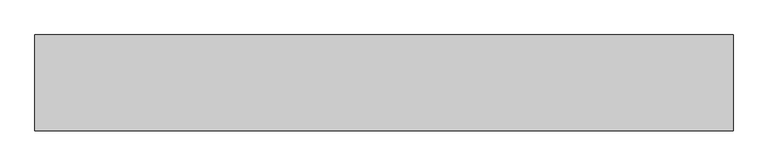
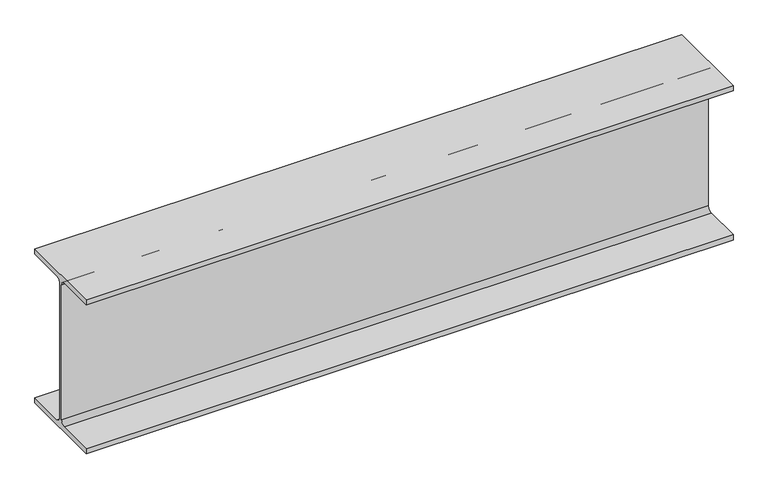
"""IFC4 building model written with IfcOpenShell, lengths in millimetres: beam geometry, Old_Steel Beam_H-KSD3502 : H_SB_ASB_H-194×150x6x9."""

from ifc_helpers import new_model, si_unit, point, frame, frame_2d, origin, place, context, project, spatial, polyline, circle_curve, trimmed, segment, composite_curve, outline, extrude, source, transform, mapped, element, save


def beam_8feac67b(model_context):
    return source(origin(), model_context, "Body", "SweptSolid", [
        extrude(outline(composite_curve([segment(polyline([(82.5, -141.5), (82.5, -151.7), (-82.5, -151.7), (-82.5, -141.5), (-11.9, -141.5)]), True, "CONTINUOUS"), segment(trimmed(circle_curve(frame_2d((-11.9, -132.6)), 8.9), [point((-11.9, -141.5))], [point((-3.0, -132.6))], True, "CARTESIAN"), True, "CONTINUOUS"), segment(polyline([(-3.0, -132.6), (-3.0, 132.6)]), True, "CONTINUOUS"), segment(trimmed(circle_curve(frame_2d((-11.9, 132.6)), 8.9), [point((-3.0, 132.6))], [point((-11.9, 141.5))], True, "CARTESIAN"), True, "CONTINUOUS"), segment(polyline([(-11.9, 141.5), (-82.5, 141.5), (-82.5, 151.7), (82.5, 151.7), (82.5, 141.5), (11.9, 141.5)]), True, "CONTINUOUS"), segment(trimmed(circle_curve(frame_2d((11.9, 132.6)), 8.9), [point((11.9, 141.5))], [point((3.0, 132.6))], True, "CARTESIAN"), True, "CONTINUOUS"), segment(polyline([(3.0, 132.6), (3.0, -132.6)]), True, "CONTINUOUS"), segment(trimmed(circle_curve(frame_2d((11.9, -132.6)), 8.9), [point((3.0, -132.6))], [point((11.9, -141.5))], True, "CARTESIAN"), True, "CONTINUOUS"), segment(polyline([(11.9, -141.5), (82.5, -141.5)]), True, "CONTINUOUS")], self_intersect=False)), frame((-601.6366265, 0.0, 0.0), z_axis=(1.0, 0.0, 0.0), x_axis=(0.0, 1.0, 0.0)), (0.0, 0.0, 1.0), 1203.2732531),
    ])


if __name__ == "__main__":
    model = new_model("IFC4")
    model_context = context("Model", 3, world=origin())
    ifc_project = project(units=[si_unit("LENGTHUNIT", "METRE", prefix="MILLI")], contexts=[model_context])
    site = spatial("IfcSite", under=ifc_project)
    building = spatial("IfcBuilding", under=site)
    placement = place(None, origin())
    beam_shape = beam_8feac67b(model_context)
    element("IfcBeam", 1, ObjectType="Old_Steel Beam_H-KSD3502 : H_SB_ASB_H-194×150x6x9", at=placement, inside=building, context=model_context, shape_type="MappedRepresentation", body=[
        mapped(beam_shape, transform((0.0, 0.0, 0.0), x_axis=(1.0, 0.0, 0.0), y_axis=(0.0, 1.0, 0.0), z_axis=(0.0, 0.0, 1.0))),
    ])
    save(model, "model.ifc")

# Revit data of these elements
# Type "Old_Steel Beam_H-KSD3502 : H_SB_ASB_H-194×150x6x9"
#   Width = 15.0 cm
#   Web Thickness = 0.6 cm
#   Web Fillet = 1.3 cm
#   Warping Constant = 43316.0 cm⁶
#   Torsional Moment of Inertia = 8.622 cm⁴
#   Torsional Modulus = 1.0 cm³
#   Section Area = 39.01 cm²
#   Plastic Modulus weak axis = 104.0 cm³
#   Plastic Modulus strong axis = 309.0 cm³
#   Perimeter = 0.95 m²/m
#   Nominal Weight = 30.60 kgf/m
#   Moment of Inertia weak axis = 507.00 cm⁴
#   Moment of Inertia strong axis = 2690.00 cm⁴
#   Height = 19.4 cm
#   Flange Thickness = 0.9 cm
#   Elastic Modulus weak axis = 67.6 cm³
#   Elastic Modulus strong axis = 277.0 cm³
#   Centroid Vertical = 9.7 cm
#   Centroid Horizontal = 7.5 cm
#   Length [instance default] = 1.5240 m
#   Structural Material [instance default] = Steel, 45-345
#   Assembly Code = ""
# Element 1 (IfcBeam, "Old_Steel Beam_H-KSD3502 : H_SB_ASB_H-194×150x6x9")
#   Structural Material = none
# Materials
#   "Steel, 45-345": class "Metal", colour RGB 189 187 185, transparency 0, Description = "Steel 345 MPa", Cost = 0
